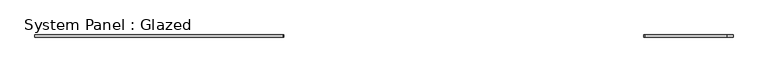
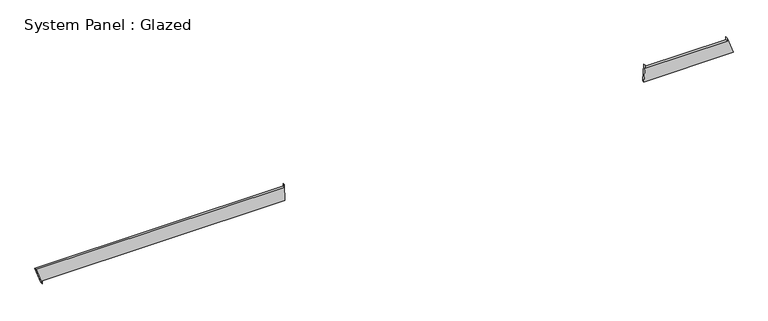
"""IFC4 building model written with IfcOpenShell, lengths in millimetres: plate geometry, System Panel : Glazed."""

from ifc_helpers import new_model, si_unit, frame, origin, place, context, project, spatial, polyline, outline, extrude, source, transform, mapped, element, save


def system_panel_glazed_6db51844(model_context):
    return source(origin(), model_context, "Body", "SweptSolid", [
        extrude(outline(polyline([(0.0, -3959.2274782), (35.3553391, -3959.2274782), (35.3553391, -1154.1262772), (234.7828866, -1159.7546078), (199.4275476, -1159.7542894), (199.4017187, -4027.8928943), (0.0, -3959.2274782)])), frame((0.0, -49.5, 0.0), z_axis=(0.0, 1.0, 0.0), x_axis=(0.0, 0.0, 1.0)), (0.0, 0.0, 1.0), 25.0),
        extrude(outline(polyline([(35.3553391, 2996.1724344), (35.3553391, 4027.8928943), (234.8289868, 3959.4017402), (199.4736478, 3959.4020585), (199.4651053, 3010.8153043), (234.8204444, 3010.814986), (35.3553391, 2996.1724344)])), frame((0.0, -49.5, 0.0), z_axis=(0.0, 1.0, 0.0), x_axis=(0.0, 0.0, 1.0)), (0.0, 0.0, 1.0), 25.0),
    ])


if __name__ == "__main__":
    model = new_model("IFC4")
    model_context = context("Model", 3, world=origin())
    ifc_project = project(units=[si_unit("LENGTHUNIT", "METRE", prefix="MILLI")], contexts=[model_context])
    site = spatial("IfcSite", under=ifc_project)
    building = spatial("IfcBuilding", under=site)
    placement = place(None, origin())
    system_panel_glazed_shape = system_panel_glazed_6db51844(model_context)
    element("IfcPlate", 1, ObjectType="System Panel : Glazed", at=placement, inside=building, context=model_context, shape_type="MappedRepresentation", body=[
        mapped(system_panel_glazed_shape, transform((0.0, 0.0, 0.0), x_axis=(1.0, 0.0, 0.0), y_axis=(0.0, 1.0, 0.0), z_axis=(0.0, 0.0, 1.0))),
    ])
    save(model, "model.ifc")

# Revit data of these elements
# Element 1 (IfcPlate, "System Panel : Glazed")
#   Materials on its faces: "Glass"
# Materials
#   "Glass": class "Glass", colour RGB 218 227 224, transparency 0.85, Description = "Soda Lime Glass", Cost = 0
